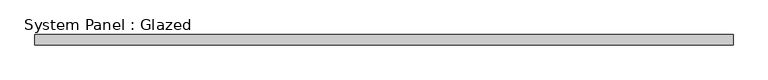
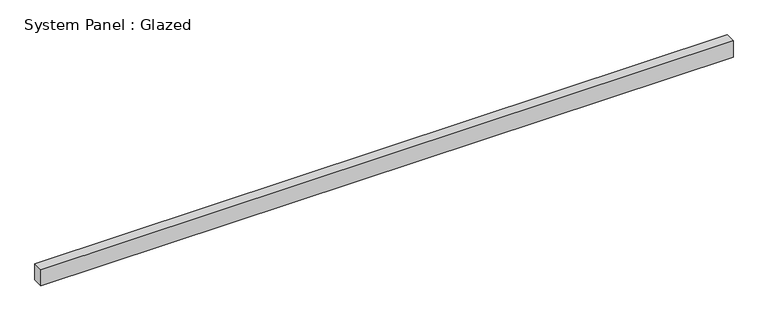
"""IFC4 building model written with IfcOpenShell, lengths in millimetres: plate geometry, System Panel : Glazed."""

from ifc_helpers import new_model, si_unit, origin, origin_with_axes, place, context, project, spatial, polyline, outline, extrude, source, transform, mapped, element, save


def system_panel_glazed_8b4ddac8(model_context):
    return source(origin(), model_context, "Body", "SweptSolid", [
        extrude(outline(polyline([(838.2000002, -44.45), (-838.2000002, -44.45), (-838.2000002, -19.05), (838.2000002, -19.05), (838.2000002, -44.45)])), origin_with_axes(), (0.0, 0.0, 1.0), 41.9143134),
    ])


if __name__ == "__main__":
    model = new_model("IFC4")
    model_context = context("Model", 3, world=origin())
    ifc_project = project(units=[si_unit("LENGTHUNIT", "METRE", prefix="MILLI")], contexts=[model_context])
    site = spatial("IfcSite", under=ifc_project)
    building = spatial("IfcBuilding", under=site)
    placement = place(None, origin())
    system_panel_glazed_shape = system_panel_glazed_8b4ddac8(model_context)
    element("IfcPlate", 1, ObjectType="System Panel : Glazed", at=placement, inside=building, context=model_context, shape_type="MappedRepresentation", body=[
        mapped(system_panel_glazed_shape, transform((0.0, 0.0, 0.0), x_axis=(1.0, 0.0, 0.0), y_axis=(0.0, 1.0, 0.0), z_axis=(0.0, 0.0, 1.0))),
    ])
    save(model, "model.ifc")

# Revit data of these elements
# Type "System Panel : Glazed"
#   Construction Type Id = "GSP4R"
#   Analytic Construction = "1/8 in Pilkington single glazing"
#   Visual Light Transmittance = 0.9
#   Solar Heat Gain Coefficient = 0.86
#   Heat Transfer Coefficient (U) = 1.18115 BTU/(h·ft²·°F)
#   Define Thermal Properties by = 1
# Element 1 (IfcPlate, "System Panel : Glazed")
#   Materials on its faces: "Glass"
# Materials
#   "Glass": class "Glass", colour RGB 0 128 192, transparency 0.75, Description = "Soda Lime Glass", Cost = 0
